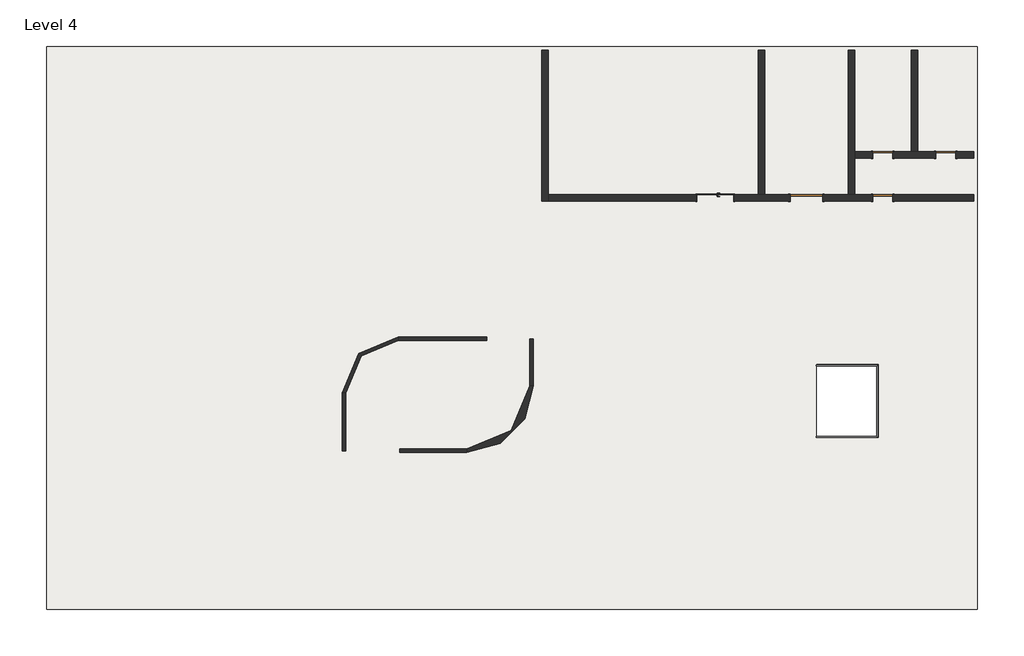
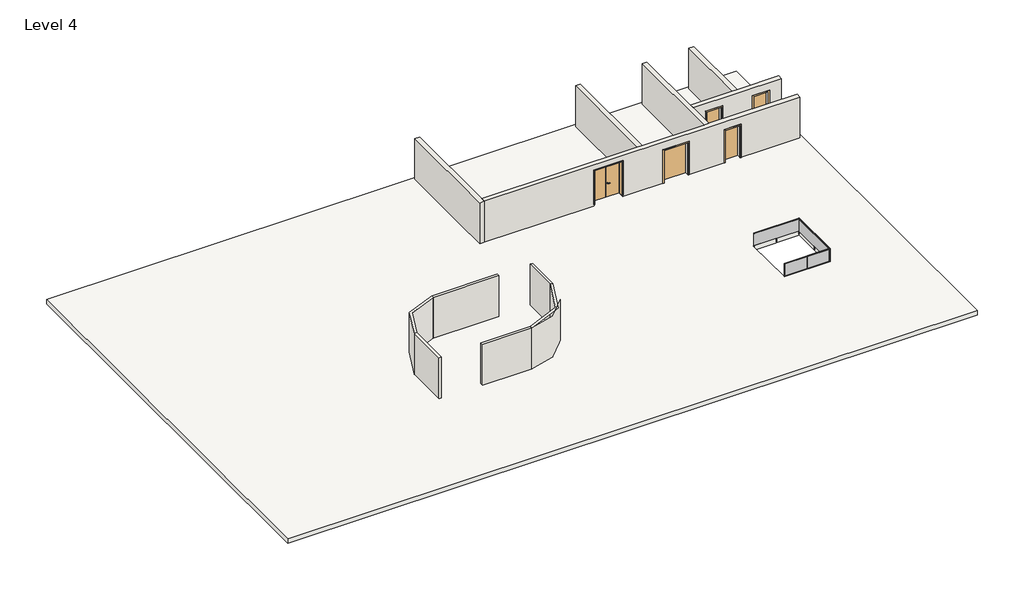
# One storey: 12 walls, 5 doors, 1 railing, 1 slab.
"""IFC4 building model written with IfcOpenShell, lengths in millimetres."""

import ifcopenshell
import ifcopenshell.guid

model = None  # the IFC model being written
_history = None  # IfcOwnerHistory: only IFC2X3 demands one
_inside = {}  # id of a spatial element -> (the spatial element, [elements in it])
_under = {}  # id of a project, library or spatial element -> (it, [spatial elements below it])
_declared = {}  # id of a project -> (the project, [libraries it declares])
_typed = {}  # id of a type object -> (the type object, [elements of that type])
_made_of = {}  # id of a material, layer set ... -> (it, [elements and type objects made of it])


def new_model(schema):
    """Start an empty IFC model of exactly this schema.

    Asked for "IFC4X3", IfcOpenShell would pick the latest addendum, in which some entities
    have other attributes; the version numbers below select the first issue.
    IFC2X3 requires an IfcOwnerHistory on every rooted entity: one is made here for all.
    """
    global model, _history
    if schema == "IFC4X3":
        model = ifcopenshell.file(schema_version=(4, 3, 0, 0))
    else:
        model = ifcopenshell.file(schema=schema)
    _inside.clear()
    _under.clear()
    _declared.clear()
    _typed.clear()
    _made_of.clear()
    _history = None
    if model.schema == "IFC2X3":
        org = make("IfcOrganization", Name="unknown")
        user = make(
            "IfcPersonAndOrganization",
            ThePerson=make("IfcPerson", FamilyName="unknown"),
            TheOrganization=org,
        )
        app = make(
            "IfcApplication",
            ApplicationDeveloper=org,
            Version="unknown",
            ApplicationFullName="unknown",
            ApplicationIdentifier="unknown",
        )
        _history = make(
            "IfcOwnerHistory",
            OwningUser=user,
            OwningApplication=app,
            ChangeAction="ADDED",
            CreationDate=0,
        )
    return model


def make(cls, **values):
    """One entity of the class cls with the attributes given. An attribute that is None is left unset."""
    return model.create_entity(
        cls, **{name: value for name, value in values.items() if value is not None}
    )


def rooted(cls, **values):
    """An entity with a GlobalId (a new one), such as an element, a storey or a relation."""
    return make(cls, GlobalId=ifcopenshell.guid.new(), OwnerHistory=_history, **values)


def si_unit(unit_type, name, prefix=None):
    """IfcSIUnit, for example si_unit("LENGTHUNIT", "METRE", prefix="MILLI")."""
    return make("IfcSIUnit", UnitType=unit_type, Prefix=prefix, Name=name)


def assignment(units):
    """IfcUnitAssignment: the units of a project."""
    return None if units is None else make("IfcUnitAssignment", Units=units)


def point(xyz):
    """IfcCartesianPoint."""
    return None if xyz is None else make("IfcCartesianPoint", Coordinates=xyz)


def direction(xyz):
    """IfcDirection."""
    return None if xyz is None else make("IfcDirection", DirectionRatios=xyz)


def frame(location, z_axis=None, x_axis=None):
    """IfcAxis2Placement3D, a coordinate frame: its origin and axes. An axis left out is left unset."""
    return make(
        "IfcAxis2Placement3D",
        Location=point(location),
        Axis=direction(z_axis),
        RefDirection=direction(x_axis),
    )


def frame_2d(location, x_axis=None):
    """IfcAxis2Placement2D, a coordinate frame in the plane: its origin and x axis."""
    return make(
        "IfcAxis2Placement2D", Location=point(location), RefDirection=direction(x_axis)
    )


def origin():
    """The frame at (0, 0, 0) with its axes left unset."""
    return frame((0.0, 0.0, 0.0))


def origin_with_axes():
    """The frame at (0, 0, 0) with the z axis (0, 0, 1) and the x axis (1, 0, 0) written out."""
    return frame((0.0, 0.0, 0.0), z_axis=(0.0, 0.0, 1.0), x_axis=(1.0, 0.0, 0.0))


def place(relative_to, where):
    """IfcLocalPlacement: puts the frame where relative to a parent placement (None: the world)."""
    return make(
        "IfcLocalPlacement", PlacementRelTo=relative_to, RelativePlacement=where
    )


def context(
    kind, dimensions, precision=None, world=None, true_north=None, identifier=None
):
    """IfcGeometricRepresentationContext, for example the 3D "Model" context."""
    return make(
        "IfcGeometricRepresentationContext",
        ContextIdentifier=identifier,
        ContextType=kind,
        CoordinateSpaceDimension=dimensions,
        Precision=precision,
        WorldCoordinateSystem=world,
        TrueNorth=true_north,
    )


def project(units=None, contexts=None):
    """IfcProject with its units and contexts."""
    return rooted(
        "IfcProject",
        Name="project",
        RepresentationContexts=contexts,
        UnitsInContext=assignment(units),
    )


def spatial(cls, under=None, at=None, **own):
    """A site, building, storey or space (cls), placed at a placement, below another one or the project."""
    s = rooted(cls, ObjectPlacement=at, **own)
    if under is not None:
        _under.setdefault(under.id(), (under, []))[1].append(s)
    return s


def polyline(points):
    """IfcPolyline through the points."""
    return make("IfcPolyline", Points=[point(p) for p in points])


def circle_curve(where, radius):
    """IfcCircle in the frame where."""
    return make("IfcCircle", Position=where, Radius=radius)


def ellipse_curve(where, semi_axis1, semi_axis2):
    """IfcEllipse in the frame where."""
    return make(
        "IfcEllipse", Position=where, SemiAxis1=semi_axis1, SemiAxis2=semi_axis2
    )


def trimmed(basis, trim1, trim2, sense, master):
    """IfcTrimmedCurve: the piece of a basis curve between two trims."""
    return make(
        "IfcTrimmedCurve",
        BasisCurve=basis,
        Trim1=trim1,
        Trim2=trim2,
        SenseAgreement=sense,
        MasterRepresentation=master,
    )


def segment(curve, same_sense, transition):
    """IfcCompositeCurveSegment."""
    return make(
        "IfcCompositeCurveSegment",
        Transition=transition,
        SameSense=same_sense,
        ParentCurve=curve,
    )


def composite_curve(segments, self_intersect=None):
    """IfcCompositeCurve: segments joined end to end."""
    return make("IfcCompositeCurve", Segments=segments, SelfIntersect=self_intersect)


def outline(outer, holes=None, kind="AREA"):
    """IfcArbitraryClosedProfileDef: a profile drawn as a closed curve; with holes, ...WithVoids."""
    if holes is None:
        return make("IfcArbitraryClosedProfileDef", ProfileType=kind, OuterCurve=outer)
    return make(
        "IfcArbitraryProfileDefWithVoids",
        ProfileType=kind,
        OuterCurve=outer,
        InnerCurves=holes,
    )


def extrude(swept, where, along, depth):
    """IfcExtrudedAreaSolid: the profile swept, set in the frame where, extruded along a direction by depth."""
    return make(
        "IfcExtrudedAreaSolid",
        SweptArea=swept,
        Position=where,
        ExtrudedDirection=direction(along),
        Depth=depth,
    )


def faces_of(points, faces, orient=None, outer=None):
    """IfcFace entities. A face is a list of loops; a loop is a list of indices into points, from 0.

    orient and outer hold one flag for each loop. By default every Orientation is true, the
    first loop of a face is its IfcFaceOuterBound and the others are IfcFaceBound.
    """
    made = []
    for i, loops in enumerate(faces):
        bounds = []
        for j, loop in enumerate(loops):
            is_outer = j == 0 if outer is None else outer[i][j]
            bounds.append(
                make(
                    "IfcFaceOuterBound" if is_outer else "IfcFaceBound",
                    Bound=make("IfcPolyLoop", Polygon=[points[k] for k in loop]),
                    Orientation=True if orient is None else orient[i][j],
                )
            )
        made.append(make("IfcFace", Bounds=bounds))
    return made


def faceted_brep(points, faces, orient=None, outer=None, voids=None):
    """IfcFacetedBrep: a solid bounded by flat faces; with voids (closed shells), ...WithVoids."""
    shared = [point(p) for p in points]
    hull = make("IfcClosedShell", CfsFaces=faces_of(shared, faces, orient, outer))
    if voids is None:
        return make("IfcFacetedBrep", Outer=hull)
    return make(
        "IfcFacetedBrepWithVoids",
        Outer=hull,
        Voids=[
            make(cls, CfsFaces=faces_of(shared, fs, o, b)) for cls, fs, o, b in voids
        ],
    )


def shape(context_of_items, identifier, shape_type, items):
    """IfcShapeRepresentation: the items that make up one representation, for example the "Body"."""
    return make(
        "IfcShapeRepresentation",
        ContextOfItems=context_of_items,
        RepresentationIdentifier=identifier,
        RepresentationType=shape_type,
        Items=items,
    )


def source(mapping_origin, context_of_items, identifier, shape_type, items):
    """IfcRepresentationMap: a shape defined once, which mapped items show again and again."""
    return make(
        "IfcRepresentationMap",
        MappingOrigin=mapping_origin,
        MappedRepresentation=shape(context_of_items, identifier, shape_type, items),
    )


def transform(
    local_origin,
    x_axis=None,
    y_axis=None,
    z_axis=None,
    scale=None,
    scale2=None,
    scale3=None,
    uniform=True,
):
    """IfcCartesianTransformationOperator3D, or its non-uniform kind. x_axis, y_axis, z_axis: its Axis1, 2, 3."""
    if uniform:
        return make(
            "IfcCartesianTransformationOperator3D",
            Axis1=direction(x_axis),
            Axis2=direction(y_axis),
            LocalOrigin=point(local_origin),
            Scale=scale,
            Axis3=direction(z_axis),
        )
    return make(
        "IfcCartesianTransformationOperator3DnonUniform",
        Axis1=direction(x_axis),
        Axis2=direction(y_axis),
        LocalOrigin=point(local_origin),
        Scale=scale,
        Axis3=direction(z_axis),
        Scale2=scale2,
        Scale3=scale3,
    )


def mapped(mapping_source, mapping_target):
    """IfcMappedItem: shows the shape of a source again, moved by a transform."""
    return make(
        "IfcMappedItem", MappingSource=mapping_source, MappingTarget=mapping_target
    )


def made_of(thing, what):
    """Note that an element or type object is made of a material, layer set ...; save() writes the relation."""
    if what is not None:
        _made_of.setdefault(what.id(), (what, []))[1].append(thing)
    return thing


def element(
    cls,
    number,
    at=None,
    inside=None,
    cuts=None,
    type_object=None,
    material=None,
    context=None,
    identifier="Body",
    shape_type=None,
    held_by="IfcProductDefinitionShape",
    body=None,
    shapes=None,
    **own,
):
    """One element of the class cls, such as IfcWall. Its Tag is "e" and its number.

    at: its placement. inside: the storey or other place that contains it. cuts: it is an
    opening in that element (IfcRelVoidsElement). A single representation is given by context,
    identifier, shape_type and body (its items); several are given by shapes. held_by: the class
    of the entity that holds the representations. save() writes the other relations.
    """
    e = rooted(cls, Tag="e%d" % number, ObjectPlacement=at, **own)
    if body is not None:
        shapes = [shape(context, identifier, shape_type, body)]
    if shapes is not None:
        e.Representation = make(held_by, Representations=shapes)
    if inside is not None:
        _inside.setdefault(inside.id(), (inside, []))[1].append(e)
    if cuts is not None:
        rooted(
            "IfcRelVoidsElement", RelatingBuildingElement=cuts, RelatedOpeningElement=e
        )
    if type_object is not None:
        _typed.setdefault(type_object.id(), (type_object, []))[1].append(e)
    return made_of(e, material)


def aggregate(whole, parts):
    """IfcRelAggregates: a whole, such as a stair, and the parts it consists of."""
    return rooted("IfcRelAggregates", RelatingObject=whole, RelatedObjects=parts)


def save(model, path):
    """Write the relations noted so far, then the file.

    IfcRelAggregates (storeys below a building ...), IfcRelContainedInSpatialStructure (elements
    in a storey), IfcRelDefinesByType, IfcRelAssociatesMaterial and IfcRelDeclares: one each for
    every whole, place, type object, material and project.
    """
    for whole, parts in _under.values():
        aggregate(whole, parts)
    for where, things in _inside.values():
        rooted(
            "IfcRelContainedInSpatialStructure",
            RelatedElements=things,
            RelatingStructure=where,
        )
    for kind, things in _typed.values():
        rooted("IfcRelDefinesByType", RelatedObjects=things, RelatingType=kind)
    for what, things in _made_of.values():
        rooted("IfcRelAssociatesMaterial", RelatedObjects=things, RelatingMaterial=what)
    for by, libraries in _declared.values():
        rooted("IfcRelDeclares", RelatingContext=by, RelatedDefinitions=libraries)
    model.write(path)


def plane_surface(at):
    """IfcPlane: the flat surface through the origin of the frame at, square to its z axis."""
    return make("IfcPlane", Position=at)


def cylinder_surface(at, radius):
    """IfcCylindricalSurface: all points at the distance radius from the z axis of the frame at."""
    return make("IfcCylindricalSurface", Position=at, Radius=radius)


def advanced_brep(points, edges, surfaces, faces):
    """IfcAdvancedBrep: a solid bounded by faces that lie on surfaces and meet in shared edges.

    An edge is (start, end): straight between two places in points (the first is 0);
    or (start, end, curve); or (start, end, curve, False) where it runs against its curve.
    A face is (place in surfaces, loops), or (place, loops, False) where it looks against
    its surface's normal. A loop lists edges by number (the first is 1), with a minus sign
    where the edge is run from its end to its start. The first loop is the outer one.
    """
    corners = [point(p) for p in points]
    vertices = [make("IfcVertexPoint", VertexGeometry=c) for c in corners]
    made = []
    for start, end, *more in edges:
        made.append(
            make(
                "IfcEdgeCurve",
                EdgeStart=vertices[start],
                EdgeEnd=vertices[end],
                EdgeGeometry=more[0] if more else make("IfcPolyline", Points=[corners[start], corners[end]]),
                SameSense=more[1] if len(more) > 1 else True,
            )
        )
    hull = []
    for where, loops, *sense in faces:
        bounds = []
        for j, loop in enumerate(loops):
            ring = [make("IfcOrientedEdge", EdgeElement=made[abs(k) - 1], Orientation=k > 0) for k in loop]
            bounds.append(
                make(
                    "IfcFaceOuterBound" if j == 0 else "IfcFaceBound",
                    Bound=make("IfcEdgeLoop", EdgeList=ring),
                    Orientation=True,
                )
            )
        hull.append(make("IfcAdvancedFace", Bounds=bounds, FaceSurface=surfaces[where], SameSense=sense[0] if sense else True))
    return make("IfcAdvancedBrep", Outer=make("IfcClosedShell", CfsFaces=hull))


def door_double_flush_variable_door_double_flush_variable_ac6c3b87(model_context):
    return source(origin(), model_context, "Body", "SolidModel", [
        advanced_brep(
        [(90.0, 139.4346141, 1000.0), (110.0, 139.4346141, 1000.0), (90.0, 69.4346141, 1000.0), (110.0, 89.4346141, 1000.0), (220.0, 69.4346141, 1000.0), (220.0, 89.4346141, 1000.0)],
        [
            (0, 1, circle_curve(frame((100.0, 139.4346141, 1000.0), z_axis=(0.0, 1.0, 0.0), x_axis=(1.0, 0.0, 0.0)), 10.0)),
            (1, 0, circle_curve(frame((100.0, 139.4346141, 1000.0), z_axis=(0.0, 1.0, 0.0), x_axis=(1.0, 0.0, 0.0)), 10.0)),
            (0, 2),
            (2, 3, ellipse_curve(frame((100.0, 79.4346141, 1000.0), z_axis=(-0.7071067811865385, 0.7071067811865565, 0.0), x_axis=(0.7071067811865563, 0.7071067811865386, 0.0)), 14.1421356, 10.0)),
            (3, 1),
            (3, 2, ellipse_curve(frame((100.0, 79.4346141, 1000.0), z_axis=(-0.7071067811865385, 0.7071067811865565, 0.0), x_axis=(0.7071067811865563, 0.7071067811865386, 0.0)), 14.1421356, 10.0)),
            (4, 5, circle_curve(frame((220.0, 79.4346141, 1000.0), z_axis=(1.0, 0.0, 0.0), x_axis=(0.0, 1.0, 0.0)), 10.0)),
            (5, 4, circle_curve(frame((220.0, 79.4346141, 1000.0), z_axis=(1.0, 0.0, 0.0), x_axis=(0.0, 1.0, 0.0)), 10.0)),
            (2, 4),
            (5, 3),
        ],
        [
            plane_surface(frame((100.0, 139.4346141, -287.7526403), z_axis=(0.0, 1.0, 0.0), x_axis=(0.0, 0.0, 1.0))),
            cylinder_surface(frame((100.0, 139.4346141, 1000.0), z_axis=(0.0, 1.0, 0.0), x_axis=(1.0, 0.0, 0.0)), 10.0),
            plane_surface(frame((220.0, 79.4346141, -287.7526403), z_axis=(1.0, 0.0, 0.0), x_axis=(0.0, 0.0, 1.0))),
            cylinder_surface(frame((100.0, 79.4346141, 1000.0), z_axis=(-1.0, 0.0, 0.0), x_axis=(0.0, 1.0, 0.0)), 10.0),
        ],
        [
            (0, [[1, 2]]),
            (1, [[-1, 3, 4, 5]]),
            (1, [[-2, -5, 6, -3]]),
            (2, [[7, 8]]),
            (3, [[-4, 9, -8, 10]]),
            (3, [[-6, -10, -7, -9]]),
        ],
    ),
        advanced_brep(
        [(110.0, 199.4346141, 1000.0), (90.0, 199.4346141, 1000.0), (110.0, 229.4346141, 1000.0), (90.0, 249.4346141, 1000.0), (220.0, 229.4346141, 1000.0), (220.0, 249.4346141, 1000.0)],
        [
            (0, 1, circle_curve(frame((100.0, 199.4346141, 1000.0), z_axis=(0.0, -1.0, 0.0), x_axis=(-1.0, 0.0, 0.0)), 10.0)),
            (1, 0, circle_curve(frame((100.0, 199.4346141, 1000.0), z_axis=(0.0, -1.0, 0.0), x_axis=(-1.0, 0.0, 0.0)), 10.0)),
            (0, 2),
            (2, 3, ellipse_curve(frame((100.0, 239.4346141, 1000.0), z_axis=(-0.7071067811865475, -0.7071067811865475, 0.0), x_axis=(0.7071067811865474, -0.7071067811865476, 0.0)), 14.1421356, 10.0)),
            (3, 1),
            (3, 2, ellipse_curve(frame((100.0, 239.4346141, 1000.0), z_axis=(-0.7071067811865475, -0.7071067811865475, 0.0), x_axis=(0.7071067811865474, -0.7071067811865476, 0.0)), 14.1421356, 10.0)),
            (4, 5, circle_curve(frame((220.0, 239.4346141, 1000.0), z_axis=(1.0, 0.0, 0.0), x_axis=(0.0, 1.0, 0.0)), 10.0)),
            (5, 4, circle_curve(frame((220.0, 239.4346141, 1000.0), z_axis=(1.0, 0.0, 0.0), x_axis=(0.0, 1.0, 0.0)), 10.0)),
            (2, 4),
            (5, 3),
        ],
        [
            plane_surface(frame((100.0, 199.4346141, -287.7526403), z_axis=(0.0, -1.0, 0.0), x_axis=(0.0, 0.0, 1.0))),
            cylinder_surface(frame((100.0, 199.4346141, 1000.0), z_axis=(0.0, -1.0, 0.0), x_axis=(-1.0, 0.0, 0.0)), 10.0),
            plane_surface(frame((220.0, 239.4346141, -287.7526403), z_axis=(1.0, 0.0, 0.0), x_axis=(0.0, 0.0, 1.0))),
            cylinder_surface(frame((100.0, 239.4346141, 1000.0), z_axis=(-1.0, 0.0, 0.0), x_axis=(0.0, 1.0, 0.0)), 10.0),
        ],
        [
            (0, [[1, 2]]),
            (1, [[-1, 3, 4, 5]]),
            (1, [[-2, -5, 6, -3]]),
            (2, [[7, 8]]),
            (3, [[-4, 9, -8, 10]]),
            (3, [[-6, -10, -7, -9]]),
        ],
    ),
        extrude(outline(composite_curve([segment(trimmed(circle_curve(frame_2d((1000.0, 100.0)), 20.0), [point((1000.0, 80.0))], [point((1000.0, 120.0))], False, "CARTESIAN"), True, "CONTINUOUS"), segment(trimmed(circle_curve(frame_2d((1000.0, 100.0)), 20.0), [point((1000.0, 120.0))], [point((1000.0, 80.0))], False, "CARTESIAN"), True, "CONTINUOUS")], self_intersect=False)), frame((0.0, 129.4346141, 0.0), z_axis=(0.0, 1.0, 0.0), x_axis=(0.0, 0.0, 1.0)), (0.0, 0.0, 1.0), 10.0),
        extrude(outline(composite_curve([segment(trimmed(circle_curve(frame_2d((1000.0, 100.0)), 20.0), [point((1000.0, 80.0))], [point((1000.0, 120.0))], False, "CARTESIAN"), True, "CONTINUOUS"), segment(trimmed(circle_curve(frame_2d((1000.0, 100.0)), 20.0), [point((1000.0, 120.0))], [point((1000.0, 80.0))], False, "CARTESIAN"), True, "CONTINUOUS")], self_intersect=False)), frame((0.0, 189.4346141, 0.0), z_axis=(0.0, 1.0, 0.0), x_axis=(0.0, 0.0, 1.0)), (0.0, 0.0, 1.0), 10.0),
        extrude(outline(polyline([(0.0, 164.4346141), (-871.25, 164.4346141), (-871.25, 189.4346141), (0.0, 189.4346141), (0.0, 164.4346141)])), frame((0.0, 0.0, 100.0), z_axis=(0.0, 0.0, 1.0), x_axis=(1.0, 0.0, 0.0)), (0.0, 0.0, 1.0), 2250.0),
        extrude(outline(polyline([(871.25, 164.4346141), (0.0, 164.4346141), (0.0, 189.4346141), (871.25, 189.4346141), (871.25, 164.4346141)])), frame((0.0, 0.0, 100.0), z_axis=(0.0, 0.0, 1.0), x_axis=(1.0, 0.0, 0.0)), (0.0, 0.0, 1.0), 2250.0),
        faceted_brep([(905.75, -150.5653859, 100.0), (856.25, -150.5653859, 100.0), (856.25, 164.4346141, 100.0), (871.25, 164.4346141, 100.0), (871.25, 189.4346141, 100.0), (905.75, 189.4346141, 100.0), (905.75, 164.4346141, 100.0), (900.75, 164.4346141, 100.0), (900.75, 184.4346141, 100.0), (876.25, 184.4346141, 100.0), (876.25, 159.4346141, 100.0), (861.25, 159.4346141, 100.0), (861.25, -145.5653859, 100.0), (900.75, -145.5653859, 100.0), (900.75, -135.5653859, 100.0), (905.75, -135.5653859, 100.0), (905.75, -150.5653859, 2384.5), (-905.75, -150.5653859, 2384.5), (-905.75, -150.5653859, 100.0), (-856.25, -150.5653859, 100.0), (-856.25, -150.5653859, 2335.0), (856.25, -150.5653859, 2335.0), (856.25, 164.4346141, 2335.0), (-856.25, 164.4346141, 2335.0), (-856.25, 164.4346141, 100.0), (-871.25, 164.4346141, 100.0), (-871.25, 164.4346141, 2350.0), (871.25, 164.4346141, 2350.0), (871.25, 189.4346141, 2350.0), (-871.25, 189.4346141, 2350.0), (-871.25, 189.4346141, 100.0), (-905.75, 189.4346141, 100.0), (-905.75, 189.4346141, 2384.5), (905.75, 189.4346141, 2384.5), (905.75, 164.4346141, 2384.5), (-905.75, 164.4346141, 2384.5), (-905.75, 164.4346141, 100.0), (-900.75, 164.4346141, 100.0), (-900.75, 164.4346141, 2379.5), (900.75, 164.4346141, 2379.5), (900.75, 184.4346141, 2379.5), (-900.75, 184.4346141, 2379.5), (-900.75, 184.4346141, 100.0), (-876.25, 184.4346141, 100.0), (-876.25, 184.4346141, 2355.0), (876.25, 184.4346141, 2355.0), (876.25, 159.4346141, 2355.0), (-876.25, 159.4346141, 2355.0), (-876.25, 159.4346141, 100.0), (-861.25, 159.4346141, 100.0), (-861.25, 159.4346141, 2340.0), (861.25, 159.4346141, 2340.0), (861.25, -145.5653859, 2340.0), (-861.25, -145.5653859, 2340.0), (-861.25, -145.5653859, 100.0), (-900.75, -145.5653859, 100.0), (-900.75, -145.5653859, 2379.5), (900.75, -145.5653859, 2379.5), (900.75, -135.5653859, 2379.5), (-900.75, -135.5653859, 2379.5), (-900.75, -135.5653859, 100.0), (-905.75, -135.5653859, 100.0), (-905.75, -135.5653859, 2384.5), (905.75, -135.5653859, 2384.5)], [[[0, 1, 2, 3, 4, 5, 6, 7, 8, 9, 10, 11, 12, 13, 14, 15]], [[1, 0, 16, 17, 18, 19, 20, 21]], [[2, 1, 21, 22]], [[3, 2, 22, 23, 24, 25, 26, 27]], [[4, 3, 27, 28]], [[5, 4, 28, 29, 30, 31, 32, 33]], [[6, 5, 33, 34]], [[7, 6, 34, 35, 36, 37, 38, 39]], [[8, 7, 39, 40]], [[9, 8, 40, 41, 42, 43, 44, 45]], [[10, 9, 45, 46]], [[11, 10, 46, 47, 48, 49, 50, 51]], [[12, 11, 51, 52]], [[13, 12, 52, 53, 54, 55, 56, 57]], [[14, 13, 57, 58]], [[15, 14, 58, 59, 60, 61, 62, 63]], [[0, 15, 63, 16]], [[17, 62, 61, 18]], [[18, 61, 60, 55, 54, 49, 48, 43, 42, 37, 36, 31, 30, 25, 24, 19]], [[23, 20, 19, 24]], [[29, 26, 25, 30]], [[35, 32, 31, 36]], [[41, 38, 37, 42]], [[47, 44, 43, 48]], [[53, 50, 49, 54]], [[59, 56, 55, 60]], [[22, 21, 20, 23]], [[28, 27, 26, 29]], [[34, 33, 32, 35]], [[40, 39, 38, 41]], [[46, 45, 44, 47]], [[52, 51, 50, 53]], [[58, 57, 56, 59]], [[16, 63, 62, 17]]]),
    ])


def m_single_flush_0915_x_2134mm_1c84716f(model_context):
    return source(origin(), model_context, "Body", "SweptSolid", [
        extrude(outline(polyline([(2210.0, -533.5), (0.0, -533.5), (0.0, -457.5), (2134.0, -457.5), (2134.0, 457.5), (0.0, 457.5), (0.0, 533.5), (2210.0, 533.5), (2210.0, -533.5)])), frame((0.0, -175.0, 0.0), z_axis=(0.0, 1.0, 0.0), x_axis=(0.0, 0.0, 1.0)), (0.0, 0.0, 1.0), 25.0),
        extrude(outline(polyline([(2210.0, 533.5), (2210.0, -533.5), (0.0, -533.5), (0.0, -457.5), (2134.0, -457.5), (2134.0, 457.5), (0.0, 457.5), (0.0, 533.5), (2210.0, 533.5)])), frame((0.0, 150.0, 0.0), z_axis=(0.0, 1.0, 0.0), x_axis=(0.0, 0.0, 1.0)), (0.0, 0.0, 1.0), 25.0),
        extrude(outline(polyline([(457.5, -99.0), (457.5, -150.0), (-457.5, -150.0), (-457.5, -99.0), (457.5, -99.0)])), origin_with_axes(), (0.0, 0.0, 1.0), 2134.0),
    ])


def m_single_flush_1500_x_2134mm_2_edebd810(model_context):
    return source(origin(), model_context, "Body", "SweptSolid", [
        extrude(outline(polyline([(2210.0, -826.0), (0.0, -826.0), (0.0, -750.0), (2134.0, -750.0), (2134.0, 750.0), (0.0, 750.0), (0.0, 826.0), (2210.0, 826.0), (2210.0, -826.0)])), frame((0.0, -175.0, 0.0), z_axis=(0.0, 1.0, 0.0), x_axis=(0.0, 0.0, 1.0)), (0.0, 0.0, 1.0), 25.0),
        extrude(outline(polyline([(2210.0, 826.0), (2210.0, -826.0), (0.0, -826.0), (0.0, -750.0), (2134.0, -750.0), (2134.0, 750.0), (0.0, 750.0), (0.0, 826.0), (2210.0, 826.0)])), frame((0.0, 150.0, 0.0), z_axis=(0.0, 1.0, 0.0), x_axis=(0.0, 0.0, 1.0)), (0.0, 0.0, 1.0), 25.0),
        extrude(outline(polyline([(750.0, -99.0), (750.0, -150.0), (-750.0, -150.0), (-750.0, -99.0), (750.0, -99.0)])), origin_with_axes(), (0.0, 0.0, 1.0), 2134.0),
    ])


def glas_mpk_39525c5c(model_context):
    return source(origin(), model_context, "Body", "SolidModel", [
        faceted_brep([(28810.8437289, 1285.374085, 9843.2628643), (28810.8437289, 1235.374085, 9843.2628643), (28810.8437289, 1235.374085, 9856.7371357), (28810.8437289, 1285.374085, 9856.7371357), (31650.8437289, 1285.374085, 9843.2628643), (31600.8437289, 1235.374085, 9843.2628643), (31600.8437289, 1235.374085, 9856.7371357), (31650.8437289, 1285.374085, 9856.7371357), (31650.8437289, -2055.3552612, 9843.2628643), (31600.8437289, -2005.3552612, 9843.2628643), (31600.8437289, -2005.3552612, 9856.7371357), (31650.8437289, -2055.3552612, 9856.7371357), (28810.8437289, -2055.3552612, 9843.2628643), (28810.8437289, -2055.3552612, 9856.7371357), (28810.8437289, -2005.3552612, 9856.7371357), (28810.8437289, -2005.3552612, 9843.2628643)], [[[0, 1, 2, 3]], [[1, 0, 4, 5]], [[2, 1, 5, 6]], [[3, 2, 6, 7]], [[0, 3, 7, 4]], [[5, 4, 8, 9]], [[6, 5, 9, 10]], [[7, 6, 10, 11]], [[4, 7, 11, 8]], [[12, 13, 14, 15]], [[9, 8, 12, 15]], [[10, 9, 15, 14]], [[11, 10, 14, 13]], [[8, 11, 13, 12]]]),
        faceted_brep([(28810.8437289, 1245.374085, 9842.8769824), (28810.8437289, 1259.566209, 9842.8769824), (28810.8437289, 1259.566209, 9042.8769824), (28810.8437289, 1245.374085, 9042.8769824), (31610.8437289, 1245.374085, 9842.8769824), (31625.0358529, 1259.566209, 9842.8769824), (31625.0358529, 1259.566209, 9042.8769824), (31610.8437289, 1245.374085, 9042.8769824), (31610.8437289, -2015.3552612, 9842.8769824), (31625.0358529, -2029.5473852, 9842.8769824), (31625.0358529, -2029.5473852, 9042.8769824), (31610.8437289, -2015.3552612, 9042.8769824), (28810.8437289, -2015.3552612, 9842.8769824), (28810.8437289, -2015.3552612, 9042.8769824), (28810.8437289, -2029.5473852, 9042.8769824), (28810.8437289, -2029.5473852, 9842.8769824)], [[[0, 1, 2, 3]], [[1, 0, 4, 5]], [[2, 1, 5, 6]], [[3, 2, 6, 7]], [[0, 3, 7, 4]], [[5, 4, 8, 9]], [[6, 5, 9, 10]], [[7, 6, 10, 11]], [[4, 7, 11, 8]], [[12, 13, 14, 15]], [[9, 8, 12, 15]], [[10, 9, 15, 14]], [[11, 10, 14, 13]], [[8, 11, 13, 12]]]),
        extrude(outline(polyline([(30242.0937289, -2030.3552612), (30242.0937289, -2055.3552612), (30217.0937289, -2055.3552612), (30217.0937289, -2030.3552612), (30242.0937289, -2030.3552612)])), frame((0.0, 0.0, 8800.0), z_axis=(0.0, 0.0, 1.0), x_axis=(1.0, 0.0, 0.0)), (0.0, 0.0, 1.0), 1043.2628643),
        extrude(outline(polyline([(31625.8437289, -372.4905881), (31650.8437289, -372.4905881), (31650.8437289, -397.4905881), (31625.8437289, -397.4905881), (31625.8437289, -372.4905881)])), frame((0.0, 0.0, 8800.0), z_axis=(0.0, 0.0, 1.0), x_axis=(1.0, 0.0, 0.0)), (0.0, 0.0, 1.0), 1043.2628643),
        extrude(outline(polyline([(30217.0937289, 1260.374085), (30217.0937289, 1285.374085), (30242.0937289, 1285.374085), (30242.0937289, 1260.374085), (30217.0937289, 1260.374085)])), frame((0.0, 0.0, 8800.0), z_axis=(0.0, 0.0, 1.0), x_axis=(1.0, 0.0, 0.0)), (0.0, 0.0, 1.0), 1043.2628643),
        extrude(outline(polyline([(31625.8437289, -2040.3552612), (31650.8437289, -2040.3552612), (31650.8437289, -2065.3552612), (31625.8437289, -2065.3552612), (31625.8437289, -2040.3552612)])), frame((0.0, 0.0, 8800.0), z_axis=(0.0, 0.0, 1.0), x_axis=(1.0, 0.0, 0.0)), (0.0, 0.0, 1.0), 1043.2628643),
        extrude(outline(polyline([(31635.8437289, 1260.374085), (31635.8437289, 1285.374085), (31660.8437289, 1285.374085), (31660.8437289, 1260.374085), (31635.8437289, 1260.374085)])), frame((0.0, 0.0, 8800.0), z_axis=(0.0, 0.0, 1.0), x_axis=(1.0, 0.0, 0.0)), (0.0, 0.0, 1.0), 1043.2628643),
        extrude(outline(polyline([(28823.3437289, -2030.3552612), (28823.3437289, -2055.3552612), (28798.3437289, -2055.3552612), (28798.3437289, -2030.3552612), (28823.3437289, -2030.3552612)])), frame((0.0, 0.0, 8800.0), z_axis=(0.0, 0.0, 1.0), x_axis=(1.0, 0.0, 0.0)), (0.0, 0.0, 1.0), 1043.2628643),
        extrude(outline(polyline([(28810.8437289, 1260.374085), (28810.8437289, 1285.374085), (28835.8437289, 1285.374085), (28835.8437289, 1260.374085), (28810.8437289, 1260.374085)])), frame((0.0, 0.0, 8800.0), z_axis=(0.0, 0.0, 1.0), x_axis=(1.0, 0.0, 0.0)), (0.0, 0.0, 1.0), 1043.2628643),
    ])


model = new_model("IFC4")

# Units and contexts
model_context = context("Model", 3, world=origin())
ifc_project = project(units=[si_unit("LENGTHUNIT", "METRE", prefix="MILLI")], contexts=[model_context])

# Site, building, storey
site = spatial("IfcSite", under=ifc_project)
building = spatial("IfcBuilding", under=site)
storey = spatial("IfcBuildingStorey", under=building, Name="Level 4", Elevation=9000.0)

# Doors
placement = place(None, origin())
door_double_flush_variable_door_double_flush_variable_shape = door_double_flush_variable_door_double_flush_variable_ac6c3b87(model_context)
element("IfcDoor", 1, ObjectType="Door Double Flush - Variable : Door Double Flush - Variable", at=placement, inside=storey, context=model_context, shape_type="MappedRepresentation", body=[
    mapped(door_double_flush_variable_door_double_flush_variable_shape, transform((24136.7471367, 8984.3231089, 9000.0), x_axis=(1.0, 0.0, 0.0), y_axis=(0.0, 1.0, 0.0), z_axis=(0.0, 0.0, 1.0))),
])
m_single_flush_0915_x_2134mm_shape = m_single_flush_0915_x_2134mm_1c84716f(model_context)
element("IfcDoor", 2, ObjectType="M_Single-Flush : 0915 x 2134mm", at=placement, inside=storey, context=model_context, shape_type="MappedRepresentation", body=[
    mapped(m_single_flush_0915_x_2134mm_shape, transform((34787.1221367, 10998.757723, 9000.0), x_axis=(-1.0, 0.0, 0.0), y_axis=(0.0, -1.0, 0.0), z_axis=(0.0, 0.0, 1.0))),
])
element("IfcDoor", 3, ObjectType="M_Single-Flush : 0915 x 2134mm", at=placement, inside=storey, context=model_context, shape_type="MappedRepresentation", body=[
    mapped(m_single_flush_0915_x_2134mm_shape, transform((31874.3721367, 10998.757723, 9000.0), x_axis=(-1.0, 0.0, 0.0), y_axis=(0.0, -1.0, 0.0), z_axis=(0.0, 0.0, 1.0))),
])
element("IfcDoor", 4, ObjectType="M_Single-Flush : 0915 x 2134mm", at=placement, inside=storey, context=model_context, shape_type="MappedRepresentation", body=[
    mapped(m_single_flush_0915_x_2134mm_shape, transform((31874.3721367, 8998.757723, 9000.0), x_axis=(-1.0, 0.0, 0.0), y_axis=(0.0, -1.0, 0.0), z_axis=(0.0, 0.0, 1.0))),
])
m_single_flush_1500_x_2134mm_2_shape = m_single_flush_1500_x_2134mm_2_edebd810(model_context)
element("IfcDoor", 5, ObjectType="M_Single-Flush : 1500 x 2134mm 2", at=placement, inside=storey, context=model_context, shape_type="MappedRepresentation", body=[
    mapped(m_single_flush_1500_x_2134mm_2_shape, transform((28342.9971367, 8998.757723, 9000.0), x_axis=(-1.0, 0.0, 0.0), y_axis=(0.0, -1.0, 0.0), z_axis=(0.0, 0.0, 1.0))),
])

# Railing
glas_mpk_shape = glas_mpk_39525c5c(model_context)
element("IfcRailing", 6, ObjectType="Glas - MPK", at=placement, inside=storey, context=model_context, shape_type="MappedRepresentation", body=[
    mapped(glas_mpk_shape, transform((0.0, 0.0, 0.0), x_axis=(1.0, 0.0, 0.0), y_axis=(0.0, 1.0, 0.0), z_axis=(0.0, 0.0, 1.0))),
])

# Slab
element("IfcSlab", 7, ObjectType="Generic 300mm", at=placement, inside=storey, context=model_context, shape_type="SweptSolid", body=[
    extrude(outline(polyline([(-6732.0028633, 15998.757723), (36243.4971367, 15998.757723), (36243.4971367, -10001.242277), (-6732.0028633, -10001.242277), (-6732.0028633, 15998.757723)]), holes=[polyline([(31663.0737371, 1305.1195288), (28813.0737371, 1305.1195288), (28813.0737371, -2055.6098174), (31663.0737371, -2055.6098174), (31663.0737371, 1305.1195288)])]), frame((0.0, 0.0, 8700.0), z_axis=(0.0, 0.0, 1.0), x_axis=(1.0, 0.0, 0.0)), (0.0, 0.0, 1.0), 300.0),
])

# Walls
element("IfcWall", 8, ObjectType="Generic - 300mm", at=placement, inside=storey, context=model_context, shape_type="Brep", body=[
    faceted_brep([(16117.9971367, 15823.757723, 9000.0), (16117.9971367, 8848.757723, 9000.0), (16117.9971367, 8848.757723, 11700.0), (16117.9971367, 15823.757723, 11700.0), (16417.9971367, 15823.757723, 9000.0), (16417.9971367, 15823.757723, 11700.0), (16417.9971367, 9148.757723, 11700.0), (16417.9971367, 8848.757723, 11700.0), (16417.9971367, 8848.757723, 9000.0), (16417.9971367, 9148.757723, 9000.0)], [[[0, 1, 2, 3]], [[4, 5, 6, 7, 8, 9]], [[1, 0, 4, 9, 8]], [[3, 2, 7, 6, 5]], [[2, 1, 8, 7]], [[0, 3, 5, 4]]]),
])
element("IfcWall", 9, ObjectType="Generic - 300mm", at=placement, inside=storey, context=model_context, shape_type="SweptSolid", body=[
    extrude(outline(polyline([(26117.9971367, 9148.757723), (26117.9971367, 15823.757723), (26417.9971367, 15823.757723), (26417.9971367, 9148.757723), (26117.9971367, 9148.757723)])), frame((0.0, 0.0, 9000.0), z_axis=(0.0, 0.0, 1.0), x_axis=(1.0, 0.0, 0.0)), (0.0, 0.0, 1.0), 2700.0),
])
element("IfcWall", 10, ObjectType="Generic - 300mm", at=placement, inside=storey, context=model_context, shape_type="Brep", body=[
    faceted_brep([(30267.9971367, 15823.757723, 9000.0), (30267.9971367, 9148.757723, 9000.0), (30267.9971367, 9148.757723, 11700.0), (30267.9971367, 15823.757723, 11700.0), (30567.9971367, 15823.757723, 9000.0), (30567.9971367, 15823.757723, 11700.0), (30567.9971367, 11148.757723, 11700.0), (30567.9971367, 10848.757723, 11700.0), (30567.9971367, 9148.757723, 11700.0), (30567.9971367, 9148.757723, 9000.0), (30567.9971367, 10848.757723, 9000.0), (30567.9971367, 11148.757723, 9000.0)], [[[0, 1, 2, 3]], [[4, 5, 6, 7, 8, 9, 10, 11]], [[1, 0, 4, 11, 10, 9]], [[3, 2, 8, 7, 6, 5]], [[2, 1, 9, 8]], [[0, 3, 5, 4]]]),
])
element("IfcWall", 11, ObjectType="Generic - 300mm", at=placement, inside=storey, context=model_context, shape_type="SweptSolid", body=[
    extrude(outline(polyline([(33180.7471367, 11148.757723), (33180.7471367, 15823.757723), (33480.7471367, 15823.757723), (33480.7471367, 11148.757723), (33180.7471367, 11148.757723)])), frame((0.0, 0.0, 9000.0), z_axis=(0.0, 0.0, 1.0), x_axis=(1.0, 0.0, 0.0)), (0.0, 0.0, 1.0), 2700.0),
])
element("IfcWall", 12, ObjectType="Generic - 300mm", at=placement, inside=storey, context=model_context, shape_type="Brep", body=[
    faceted_brep([(16417.9971367, 9148.757723, 11700.0), (26117.9971367, 9148.757723, 11700.0), (26417.9971367, 9148.757723, 11700.0), (30267.9971367, 9148.757723, 11700.0), (30567.9971367, 9148.757723, 11700.0), (36068.4971367, 9148.757723, 11700.0), (36068.4971367, 9148.757723, 9000.0), (32331.8721367, 9148.757723, 9000.0), (32331.8721367, 9148.757723, 11134.0), (31416.8721367, 9148.757723, 11134.0), (31416.8721367, 9148.757723, 9000.0), (30567.9971367, 9148.757723, 9000.0), (30267.9971367, 9148.757723, 9000.0), (29092.9971367, 9148.757723, 9000.0), (29092.9971367, 9148.757723, 11134.0), (27592.9971367, 9148.757723, 11134.0), (27592.9971367, 9148.757723, 9000.0), (26417.9971367, 9148.757723, 9000.0), (26117.9971367, 9148.757723, 9000.0), (25017.9971367, 9148.757723, 9000.0), (25017.9971367, 9148.757723, 11360.0), (23255.4971367, 9148.757723, 11360.0), (23255.4971367, 9148.757723, 9000.0), (16417.9971367, 9148.757723, 9000.0), (36068.4971367, 8848.757723, 11700.0), (16417.9971367, 8848.757723, 11700.0), (16417.9971367, 8848.757723, 9000.0), (23255.4971367, 8848.757723, 9000.0), (23255.4971367, 8848.757723, 11360.0), (25017.9971367, 8848.757723, 11360.0), (25017.9971367, 8848.757723, 9000.0), (27592.9971367, 8848.757723, 9000.0), (27592.9971367, 8848.757723, 11134.0), (29092.9971367, 8848.757723, 11134.0), (29092.9971367, 8848.757723, 9000.0), (31416.8721367, 8848.757723, 9000.0), (31416.8721367, 8848.757723, 11134.0), (32331.8721367, 8848.757723, 11134.0), (32331.8721367, 8848.757723, 9000.0), (36068.4971367, 8848.757723, 9000.0)], [[[0, 1, 2, 3, 4, 5, 6, 7, 8, 9, 10, 11, 12, 13, 14, 15, 16, 17, 18, 19, 20, 21, 22, 23]], [[24, 25, 26, 27, 28, 29, 30, 31, 32, 33, 34, 35, 36, 37, 38, 39]], [[26, 23, 22, 27]], [[10, 35, 34, 13, 12, 11]], [[38, 7, 6, 39]], [[16, 31, 30, 19, 18, 17]], [[5, 4, 3, 2, 1, 0, 25, 24]], [[0, 23, 26, 25]], [[36, 35, 10, 9]], [[37, 36, 9, 8]], [[38, 37, 8, 7]], [[32, 31, 16, 15]], [[33, 32, 15, 14]], [[34, 33, 14, 13]], [[29, 20, 19, 30]], [[20, 29, 28, 21]], [[21, 28, 27, 22]], [[6, 5, 24, 39]]]),
])
element("IfcWall", 13, ObjectType="Generic - 300mm", at=placement, inside=storey, context=model_context, shape_type="Brep", body=[
    faceted_brep([(31416.8721367, 11148.757723, 11134.0), (31416.8721367, 11148.757723, 9000.0), (30567.9971367, 11148.757723, 9000.0), (30567.9971367, 11148.757723, 11700.0), (33180.7471367, 11148.757723, 11700.0), (33480.7471367, 11148.757723, 11700.0), (36068.4971367, 11148.757723, 11700.0), (36068.4971367, 11148.757723, 9000.0), (35244.6221367, 11148.757723, 9000.0), (35244.6221367, 11148.757723, 11134.0), (34329.6221367, 11148.757723, 11134.0), (34329.6221367, 11148.757723, 9000.0), (33480.7471367, 11148.757723, 9000.0), (33180.7471367, 11148.757723, 9000.0), (32331.8721367, 11148.757723, 9000.0), (32331.8721367, 11148.757723, 11134.0), (30567.9971367, 10848.757723, 9000.0), (31416.8721367, 10848.757723, 9000.0), (31416.8721367, 10848.757723, 11134.0), (32331.8721367, 10848.757723, 11134.0), (32331.8721367, 10848.757723, 9000.0), (34329.6221367, 10848.757723, 9000.0), (34329.6221367, 10848.757723, 11134.0), (35244.6221367, 10848.757723, 11134.0), (35244.6221367, 10848.757723, 9000.0), (36068.4971367, 10848.757723, 9000.0), (36068.4971367, 10848.757723, 11700.0), (30567.9971367, 10848.757723, 11700.0)], [[[0, 1, 2, 3, 4, 5, 6, 7, 8, 9, 10, 11, 12, 13, 14, 15]], [[16, 17, 18, 19, 20, 21, 22, 23, 24, 25, 26, 27]], [[8, 7, 25, 24]], [[2, 1, 17, 16]], [[14, 13, 12, 11, 21, 20]], [[6, 5, 4, 3, 27, 26]], [[3, 2, 16, 27]], [[22, 21, 11, 10]], [[23, 22, 10, 9]], [[24, 23, 9, 8]], [[18, 17, 1, 0]], [[19, 18, 0, 15]], [[20, 19, 15, 14]], [[7, 6, 26, 25]]]),
])
element("IfcWall", 14, ObjectType="Interior - Blockwork 140", at=placement, inside=storey, context=model_context, shape_type="SweptSolid", body=[
    extrude(outline(polyline([(13583.5160614, 2407.0363043), (9501.5160614, 2407.0363043), (9501.5160614, 2571.0363043), (13583.5160614, 2571.0363043), (13583.5160614, 2407.0363043)])), frame((0.0, 0.0, 9000.0), z_axis=(0.0, 0.0, 1.0), x_axis=(1.0, 0.0, 0.0)), (0.0, 0.0, 1.0), 2700.0),
])
element("IfcWall", 15, ObjectType="Interior - Blockwork 140", at=placement, inside=storey, context=model_context, shape_type="SweptSolid", body=[
    extrude(outline(polyline([(7083.5160614, -10.9636957), (7083.5160614, -2674.9636957), (6919.5160614, -2674.9636957), (6919.5160614, -10.9636957), (7083.5160614, -10.9636957)])), frame((0.0, 0.0, 9000.0), z_axis=(0.0, 0.0, 1.0), x_axis=(1.0, 0.0, 0.0)), (0.0, 0.0, 1.0), 2700.0),
])
element("IfcWall", 16, ObjectType="Interior - Blockwork 140", at=placement, inside=storey, context=model_context, shape_type="SweptSolid", body=[
    extrude(outline(polyline([(9583.5160614, -2592.9636957), (12665.5160614, -2592.9636957), (12665.5160614, -2756.9636957), (9583.5160614, -2756.9636957), (9583.5160614, -2592.9636957)])), frame((0.0, 0.0, 9000.0), z_axis=(0.0, 0.0, 1.0), x_axis=(1.0, 0.0, 0.0)), (0.0, 0.0, 1.0), 2700.0),
])
element("IfcWall", 17, ObjectType="Interior - Blockwork 140", at=placement, inside=storey, context=model_context, shape_type="SweptSolid", body=[
    extrude(outline(polyline([(15583.5160614, 325.0363043), (15583.5160614, 2489.0363043), (15747.5160614, 2489.0363043), (15747.5160614, 325.0363043), (15583.5160614, 325.0363043)])), frame((0.0, 0.0, 9000.0), z_axis=(0.0, 0.0, 1.0), x_axis=(1.0, 0.0, 0.0)), (0.0, 0.0, 1.0), 2700.0),
])
element("IfcWall", 18, ObjectType="Interior - Blockwork 140", at=placement, inside=storey, context=model_context, shape_type="SweptSolid", body=[
    extrude(outline(composite_curve([segment(polyline([(7083.5160614, -10.9636957), (6919.5160614, -10.9636957)]), True, "CONTINUOUS"), segment(trimmed(circle_curve(frame_2d((9501.5160614, -10.9636957)), 2582.0), [point((6919.5160614, -10.9636957))], [point((9501.5160614, 2571.0363043))], False, "CARTESIAN"), True, "CONTINUOUS"), segment(polyline([(9501.5160614, 2571.0363043), (9501.5160614, 2407.0363043)]), True, "CONTINUOUS"), segment(trimmed(circle_curve(frame_2d((9501.5160614, -10.9636957)), 2418.0), [point((9501.5160614, 2407.0363043))], [point((7083.5160614, -10.9636957))], True, "CARTESIAN"), True, "CONTINUOUS")], self_intersect=False)), frame((0.0, 0.0, 9000.0), z_axis=(0.0, 0.0, 1.0), x_axis=(1.0, 0.0, 0.0)), (0.0, 0.0, 1.0), 2700.0),
])
element("IfcWall", 19, ObjectType="Interior - Blockwork 140", at=placement, inside=storey, context=model_context, shape_type="SweptSolid", body=[
    extrude(outline(composite_curve([segment(polyline([(15583.5160614, 325.0363043), (15747.5160614, 325.0363043)]), True, "CONTINUOUS"), segment(trimmed(circle_curve(frame_2d((12665.5160614, 325.0363043)), 3082.0), [point((15747.5160614, 325.0363043))], [point((12665.5160614, -2756.9636957))], False, "CARTESIAN"), True, "CONTINUOUS"), segment(polyline([(12665.5160614, -2756.9636957), (12665.5160614, -2592.9636957)]), True, "CONTINUOUS"), segment(trimmed(circle_curve(frame_2d((12665.5160614, 325.0363043)), 2918.0), [point((12665.5160614, -2592.9636957))], [point((15583.5160614, 325.0363043))], True, "CARTESIAN"), True, "CONTINUOUS")], self_intersect=False)), frame((0.0, 0.0, 9000.0), z_axis=(0.0, 0.0, 1.0), x_axis=(1.0, 0.0, 0.0)), (0.0, 0.0, 1.0), 2700.0),
])

save(model, "model.ifc")

# Revit data of these elements
# Project information
#   Project Issue Date = "Issue Date"
#   Project Status = "Project Status"
#   Client Name = "Owner"
#   Project Address = "Enter address here"
#   Project Name = "Project Name"
#   Project Number = "Project Number"
#   Document GUID = "c2a387e2-990c-40c9-8e77-3791c5d4ece9"
# Grids (mm)
#   "1": line (-6732.003, -17149.184) -> (-6732.003, 20035.144)
#   "2": line (-3732.003, -17149.184) -> (-3732.003, 20035.144)
#   "3": line (6267.997, -17149.184) -> (6267.997, 20035.144)
#   "4": line (16267.997, -17149.184) -> (16267.997, 20035.144)
#   "5": line (26267.997, -17149.184) -> (26267.997, 20035.144)
#   "6": line (36243.497, -17149.184) -> (36243.497, 20035.144)
#   "A": line (42039.58, 15998.758) -> (-12000.946, 15998.758)
#   "B": line (42039.58, 12998.758) -> (-12000.946, 12998.758)
#   "C": line (42039.58, 2998.758) -> (-12000.946, 2998.758)
#   "D": line (42039.58, -7001.242) -> (-12000.946, -7001.242)
#   "E": line (42039.58, -10001.242) -> (-12000.946, -10001.242)
# Type "Door Double Flush - Variable : Door Double Flush - Variable"
#   Type Mark = "33"
#   Operation = "DoubleDoorSingleSwing"
#   Keynote = "16.03"
#   Rough Width [instance default] = 2.010 m
#   Rough Height [instance default] = 2.360 m
#   Doorhandle Height = 0.900 m
#   Height [instance default] = 2.260 m
#   Sill Height [instance default] = 0.100 m
#   Width [instance default] = 2.010 m
#   Visibility [instance default] = yes
#   Doorhandle choose [instance default] = element 138974
#   Doorhandle [instance default] = Metal _ Chrome
#   Door [instance default] = Door - Wood
#   Frame [instance default] = Door - Wood
#   Function = (empty or 0)
#   Wall Closure = (empty or 0)
#   Assembly Code = ""
# Type "M_Single-Flush : 0915 x 2134mm"
#   Type Mark = "20"
#   Thickness = 0.051 m
#   Height = 2.134 m
#   Trim Projection Ext = 0.025 m
#   Trim Projection Int = 0.025 m
#   Trim Width = 0.076 m
#   Width = 0.915 m
#   Door Material = Door - Panel
#   Frame Material = Door - Frame
#   Function = (empty or 0)
#   Wall Closure = (empty or 0)
# Type "M_Single-Flush : 1500 x 2134mm 2"
#   Type Mark = "34"
#   Thickness = 0.051 m
#   Height = 2.134 m
#   Trim Projection Ext = 0.025 m
#   Trim Projection Int = 0.025 m
#   Trim Width = 0.076 m
#   Width = 1.500 m
#   Door Material = Door - Panel
#   Frame Material = Door - Frame
#   Function = (empty or 0)
#   Wall Closure = (empty or 0)
# Type "Glas - MPK"
#   built-in parameter 1008619 = -0.0410105 (stored number, unit not read)
#   built-in parameter 1008612 = 0.019685 (stored number, unit not read)
#   built-in parameter 1008611 = 0.0984252 (stored number, unit not read)
#   built-in parameter 1008609 = 6.56168 (stored number, unit not read)
#   built-in parameter 1008604 = 0.19685 (stored number, unit not read)
#   built-in parameter 1008603 = 0.164042 (stored number, unit not read)
#   Railing Height = 0.865 m
#   built-in parameter 1008630 = 2
#   built-in parameter 1008610 = 1
#   built-in parameter 1008605 = 1
# Type "Generic 300mm"
#   Function = 0
#   Layers, outside or top first: 0.300 m no material (function 1)
# Type "Generic - 300mm"
#   Layers, outside or top first: 0.300 m no material (function 1)
# Type "Interior - Blockwork 140"
#   Layers, outside or top first: 0.012 m "Plasterboard" (function 5); 0.140 m "Masonry - Concrete Block" (function 1); 0.012 m "Plasterboard" (function 5)
# Element 1 (IfcDoor, "Door Double Flush - Variable : Door Double Flush - Variable")
#   Width = 1.7625 m
#   Sill Height = 0.100 m
#   Rough Width = 1.7625 m
#   Rough Height = 2.360 m
#   Height = 2.260 m
#   Visibility = yes
#   Frame = Door - Wood
#   Doorhandle choose = element 138974
#   Doorhandle = Metal _ Chrome
#   Door = Door - Wood
#   Phase Created = New Construction
#   Materials on its faces: "Door - Wood", "Metal _ Chrome"
# Elements 2, 3, 4 (IfcDoor, "M_Single-Flush : 0915 x 2134mm")
#   Phase Created = New Construction
#   Materials on its faces: "Door - Frame", "Door - Panel"
# Element 5 (IfcDoor, "M_Single-Flush : 1500 x 2134mm 2")
#   Phase Created = New Construction
#   Materials on its faces: "Door - Frame", "Door - Panel"
# Element 6 (IfcRailing, "Glas - MPK")
#   Phase Created = New Construction
#   Materials on its faces: "Metal - Aluminum", "Window - Glass"
# Element 7 (IfcSlab, "Generic 300mm")
#   built-in parameter 1001955 = 3.14159 (stored number, unit not read)
#   Height Offset From Level = 0.000 m
#   Phase Created = New Construction
#   Materials on its faces: "Default Floor"
# Elements 8, 9, 10, 11, 12, 13 (IfcWall, "Generic - 300mm")
#   Top Offset = -0.300 m
#   Base Offset = 0.000 m
#   wall height = 2.700 m
#   Phase Created = New Construction
#   Base Constraint = Level 4
#   Top Constraint = Level 5
#   Materials on its faces: "Default Wall"
# Elements 14, 15, 16, 17 (IfcWall, "Interior - Blockwork 140")
#   Top Offset = -0.300 m
#   Base Offset = 0.000 m
#   wall height = 2.700 m
#   Phase Created = New Construction
#   Base Constraint = Level 4
#   Top Constraint = Level 5
#   Materials on its faces: "Default Wall", "Plasterboard"
# Elements 18, 19 (IfcWall, "Interior - Blockwork 140")
#   Top Offset = -0.300 m
#   Base Offset = 0.000 m
#   Unconnected Height = 4.000 m
#   wall height = 2.700 m
#   Phase Created = New Construction
#   Materials on its faces: "Default Wall", "Plasterboard"
# Materials
#   "Metal _ Chrome": class "Metall", colour RGB 247 247 247, transparency 0
#   "Door - Wood": class "Unassigned", colour RGB 114 94 79, transparency 0
#   "Door - Panel": class "Wood", colour RGB 210 159 95, transparency 0
#   "Door - Frame": class "Miscellaneous", colour RGB 118 70 51, transparency 0
#   "Plasterboard": class "Drywall", colour RGB 249 249 249, transparency 0, Description = "Interior finish"
#   "Masonry - Concrete Block": class "Concrete", colour RGB 181 181 181, transparency 0
#   "Metal - Aluminum": class "Unassigned", colour RGB 247 247 247, transparency 0, Comments = "Rendering appearance not upgraded "
#   "Window - Glass": class "Glas", colour RGB 128 128 255, transparency 0.75
#   "Default Floor": class "Miscellaneous", colour RGB 127 127 127, transparency 0
#   "Default Wall": class "Miscellaneous", colour RGB 128 128 128, transparency 0
